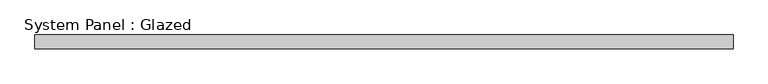
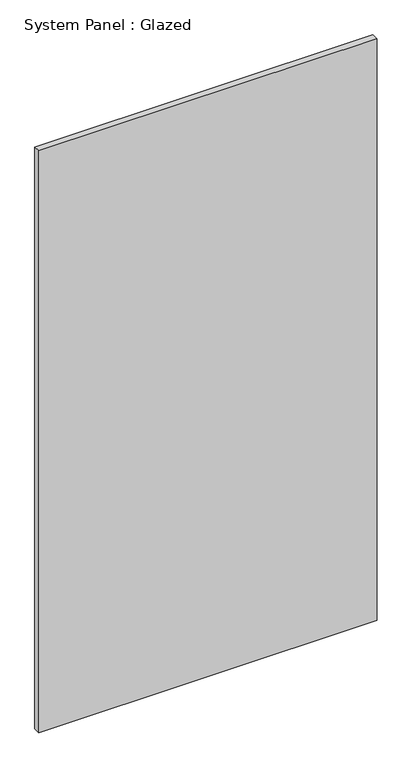
"""IFC4 building model written with IfcOpenShell, lengths in millimetres: plate geometry, System Panel : Glazed."""

from ifc_helpers import new_model, si_unit, origin, origin_with_axes, place, context, project, spatial, polyline, outline, extrude, source, transform, mapped, element, save


def system_panel_glazed_fd68b2ce(model_context):
    return source(origin(), model_context, "Body", "SweptSolid", [
        extrude(outline(polyline([(639.2857142, 24.5), (-639.2857142, 24.5), (-639.2857142, 49.5), (639.2857142, 49.5), (639.2857142, 24.5)])), origin_with_axes(), (0.0, 0.0, 1.0), 2325.0),
    ])


if __name__ == "__main__":
    model = new_model("IFC4")
    model_context = context("Model", 3, world=origin())
    ifc_project = project(units=[si_unit("LENGTHUNIT", "METRE", prefix="MILLI")], contexts=[model_context])
    site = spatial("IfcSite", under=ifc_project)
    building = spatial("IfcBuilding", under=site)
    placement = place(None, origin())
    system_panel_glazed_shape = system_panel_glazed_fd68b2ce(model_context)
    element("IfcPlate", 1, ObjectType="System Panel : Glazed", at=placement, inside=building, context=model_context, shape_type="MappedRepresentation", body=[
        mapped(system_panel_glazed_shape, transform((0.0, 0.0, 0.0), x_axis=(1.0, 0.0, 0.0), y_axis=(0.0, 1.0, 0.0), z_axis=(0.0, 0.0, 1.0))),
    ])
    save(model, "model.ifc")

# Revit data of these elements
# Type "System Panel : Glazed"
#   Construction Type Id = "GSP4R"
#   Analytic Construction = "1/8 in Pilkington single glazing"
#   Visual Light Transmittance = 0.9
#   Solar Heat Gain Coefficient = 0.86
#   Heat Transfer Coefficient (U) = 6.7069 W/(m²·K)
#   Define Thermal Properties by = 1
# Element 1 (IfcPlate, "System Panel : Glazed")
#   Materials on its faces: "Glass"
# Materials
#   "Glass": class "Glass", colour RGB 0 128 192, transparency 0.75, Description = "Soda Lime Glass", Cost = 0
